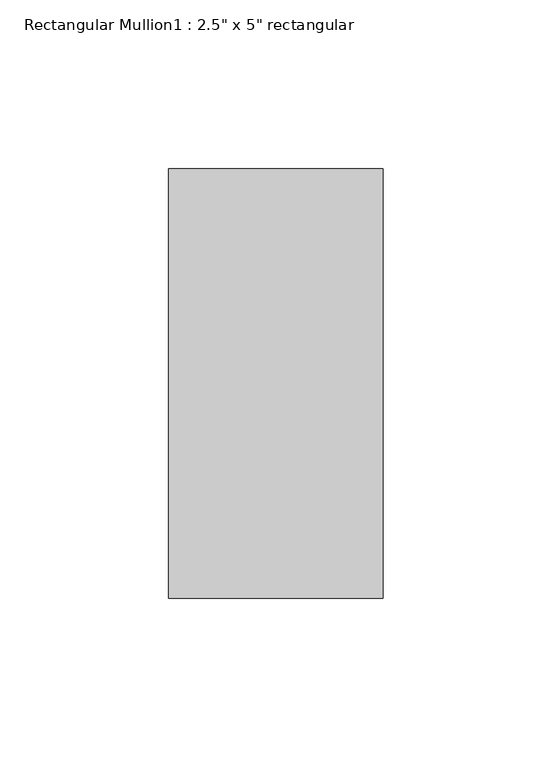
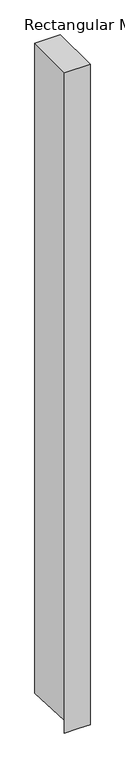
"""IFC4 building model written with IfcOpenShell, lengths in millimetres: member geometry."""

import ifcopenshell
import ifcopenshell.guid

model = None  # the IFC model being written
_history = None  # IfcOwnerHistory: only IFC2X3 demands one
_inside = {}  # id of a spatial element -> (the spatial element, [elements in it])
_under = {}  # id of a project, library or spatial element -> (it, [spatial elements below it])
_declared = {}  # id of a project -> (the project, [libraries it declares])
_typed = {}  # id of a type object -> (the type object, [elements of that type])
_made_of = {}  # id of a material, layer set ... -> (it, [elements and type objects made of it])


def new_model(schema):
    """Start an empty IFC model of exactly this schema.

    Asked for "IFC4X3", IfcOpenShell would pick the latest addendum, in which some entities
    have other attributes; the version numbers below select the first issue.
    IFC2X3 requires an IfcOwnerHistory on every rooted entity: one is made here for all.
    """
    global model, _history
    if schema == "IFC4X3":
        model = ifcopenshell.file(schema_version=(4, 3, 0, 0))
    else:
        model = ifcopenshell.file(schema=schema)
    _inside.clear()
    _under.clear()
    _declared.clear()
    _typed.clear()
    _made_of.clear()
    _history = None
    if model.schema == "IFC2X3":
        org = make("IfcOrganization", Name="unknown")
        user = make(
            "IfcPersonAndOrganization",
            ThePerson=make("IfcPerson", FamilyName="unknown"),
            TheOrganization=org,
        )
        app = make(
            "IfcApplication",
            ApplicationDeveloper=org,
            Version="unknown",
            ApplicationFullName="unknown",
            ApplicationIdentifier="unknown",
        )
        _history = make(
            "IfcOwnerHistory",
            OwningUser=user,
            OwningApplication=app,
            ChangeAction="ADDED",
            CreationDate=0,
        )
    return model


def make(cls, **values):
    """One entity of the class cls with the attributes given. An attribute that is None is left unset."""
    return model.create_entity(
        cls, **{name: value for name, value in values.items() if value is not None}
    )


def rooted(cls, **values):
    """An entity with a GlobalId (a new one), such as an element, a storey or a relation."""
    return make(cls, GlobalId=ifcopenshell.guid.new(), OwnerHistory=_history, **values)


def si_unit(unit_type, name, prefix=None):
    """IfcSIUnit, for example si_unit("LENGTHUNIT", "METRE", prefix="MILLI")."""
    return make("IfcSIUnit", UnitType=unit_type, Prefix=prefix, Name=name)


def assignment(units):
    """IfcUnitAssignment: the units of a project."""
    return None if units is None else make("IfcUnitAssignment", Units=units)


def point(xyz):
    """IfcCartesianPoint."""
    return None if xyz is None else make("IfcCartesianPoint", Coordinates=xyz)


def direction(xyz):
    """IfcDirection."""
    return None if xyz is None else make("IfcDirection", DirectionRatios=xyz)


def frame(location, z_axis=None, x_axis=None):
    """IfcAxis2Placement3D, a coordinate frame: its origin and axes. An axis left out is left unset."""
    return make(
        "IfcAxis2Placement3D",
        Location=point(location),
        Axis=direction(z_axis),
        RefDirection=direction(x_axis),
    )


def origin():
    """The frame at (0, 0, 0) with its axes left unset."""
    return frame((0.0, 0.0, 0.0))


def place(relative_to, where):
    """IfcLocalPlacement: puts the frame where relative to a parent placement (None: the world)."""
    return make(
        "IfcLocalPlacement", PlacementRelTo=relative_to, RelativePlacement=where
    )


def context(
    kind, dimensions, precision=None, world=None, true_north=None, identifier=None
):
    """IfcGeometricRepresentationContext, for example the 3D "Model" context."""
    return make(
        "IfcGeometricRepresentationContext",
        ContextIdentifier=identifier,
        ContextType=kind,
        CoordinateSpaceDimension=dimensions,
        Precision=precision,
        WorldCoordinateSystem=world,
        TrueNorth=true_north,
    )


def project(units=None, contexts=None):
    """IfcProject with its units and contexts."""
    return rooted(
        "IfcProject",
        Name="project",
        RepresentationContexts=contexts,
        UnitsInContext=assignment(units),
    )


def spatial(cls, under=None, at=None, **own):
    """A site, building, storey or space (cls), placed at a placement, below another one or the project."""
    s = rooted(cls, ObjectPlacement=at, **own)
    if under is not None:
        _under.setdefault(under.id(), (under, []))[1].append(s)
    return s


def faces_of(points, faces, orient=None, outer=None):
    """IfcFace entities. A face is a list of loops; a loop is a list of indices into points, from 0.

    orient and outer hold one flag for each loop. By default every Orientation is true, the
    first loop of a face is its IfcFaceOuterBound and the others are IfcFaceBound.
    """
    made = []
    for i, loops in enumerate(faces):
        bounds = []
        for j, loop in enumerate(loops):
            is_outer = j == 0 if outer is None else outer[i][j]
            bounds.append(
                make(
                    "IfcFaceOuterBound" if is_outer else "IfcFaceBound",
                    Bound=make("IfcPolyLoop", Polygon=[points[k] for k in loop]),
                    Orientation=True if orient is None else orient[i][j],
                )
            )
        made.append(make("IfcFace", Bounds=bounds))
    return made


def faceted_brep(points, faces, orient=None, outer=None, voids=None):
    """IfcFacetedBrep: a solid bounded by flat faces; with voids (closed shells), ...WithVoids."""
    shared = [point(p) for p in points]
    hull = make("IfcClosedShell", CfsFaces=faces_of(shared, faces, orient, outer))
    if voids is None:
        return make("IfcFacetedBrep", Outer=hull)
    return make(
        "IfcFacetedBrepWithVoids",
        Outer=hull,
        Voids=[
            make(cls, CfsFaces=faces_of(shared, fs, o, b)) for cls, fs, o, b in voids
        ],
    )


def shape(context_of_items, identifier, shape_type, items):
    """IfcShapeRepresentation: the items that make up one representation, for example the "Body"."""
    return make(
        "IfcShapeRepresentation",
        ContextOfItems=context_of_items,
        RepresentationIdentifier=identifier,
        RepresentationType=shape_type,
        Items=items,
    )


def source(mapping_origin, context_of_items, identifier, shape_type, items):
    """IfcRepresentationMap: a shape defined once, which mapped items show again and again."""
    return make(
        "IfcRepresentationMap",
        MappingOrigin=mapping_origin,
        MappedRepresentation=shape(context_of_items, identifier, shape_type, items),
    )


def transform(
    local_origin,
    x_axis=None,
    y_axis=None,
    z_axis=None,
    scale=None,
    scale2=None,
    scale3=None,
    uniform=True,
):
    """IfcCartesianTransformationOperator3D, or its non-uniform kind. x_axis, y_axis, z_axis: its Axis1, 2, 3."""
    if uniform:
        return make(
            "IfcCartesianTransformationOperator3D",
            Axis1=direction(x_axis),
            Axis2=direction(y_axis),
            LocalOrigin=point(local_origin),
            Scale=scale,
            Axis3=direction(z_axis),
        )
    return make(
        "IfcCartesianTransformationOperator3DnonUniform",
        Axis1=direction(x_axis),
        Axis2=direction(y_axis),
        LocalOrigin=point(local_origin),
        Scale=scale,
        Axis3=direction(z_axis),
        Scale2=scale2,
        Scale3=scale3,
    )


def mapped(mapping_source, mapping_target):
    """IfcMappedItem: shows the shape of a source again, moved by a transform."""
    return make(
        "IfcMappedItem", MappingSource=mapping_source, MappingTarget=mapping_target
    )


def made_of(thing, what):
    """Note that an element or type object is made of a material, layer set ...; save() writes the relation."""
    if what is not None:
        _made_of.setdefault(what.id(), (what, []))[1].append(thing)
    return thing


def element(
    cls,
    number,
    at=None,
    inside=None,
    cuts=None,
    type_object=None,
    material=None,
    context=None,
    identifier="Body",
    shape_type=None,
    held_by="IfcProductDefinitionShape",
    body=None,
    shapes=None,
    **own,
):
    """One element of the class cls, such as IfcWall. Its Tag is "e" and its number.

    at: its placement. inside: the storey or other place that contains it. cuts: it is an
    opening in that element (IfcRelVoidsElement). A single representation is given by context,
    identifier, shape_type and body (its items); several are given by shapes. held_by: the class
    of the entity that holds the representations. save() writes the other relations.
    """
    e = rooted(cls, Tag="e%d" % number, ObjectPlacement=at, **own)
    if body is not None:
        shapes = [shape(context, identifier, shape_type, body)]
    if shapes is not None:
        e.Representation = make(held_by, Representations=shapes)
    if inside is not None:
        _inside.setdefault(inside.id(), (inside, []))[1].append(e)
    if cuts is not None:
        rooted(
            "IfcRelVoidsElement", RelatingBuildingElement=cuts, RelatedOpeningElement=e
        )
    if type_object is not None:
        _typed.setdefault(type_object.id(), (type_object, []))[1].append(e)
    return made_of(e, material)


def aggregate(whole, parts):
    """IfcRelAggregates: a whole, such as a stair, and the parts it consists of."""
    return rooted("IfcRelAggregates", RelatingObject=whole, RelatedObjects=parts)


def save(model, path):
    """Write the relations noted so far, then the file.

    IfcRelAggregates (storeys below a building ...), IfcRelContainedInSpatialStructure (elements
    in a storey), IfcRelDefinesByType, IfcRelAssociatesMaterial and IfcRelDeclares: one each for
    every whole, place, type object, material and project.
    """
    for whole, parts in _under.values():
        aggregate(whole, parts)
    for where, things in _inside.values():
        rooted(
            "IfcRelContainedInSpatialStructure",
            RelatedElements=things,
            RelatingStructure=where,
        )
    for kind, things in _typed.values():
        rooted("IfcRelDefinesByType", RelatedObjects=things, RelatingType=kind)
    for what, things in _made_of.values():
        rooted("IfcRelAssociatesMaterial", RelatedObjects=things, RelatingMaterial=what)
    for by, libraries in _declared.values():
        rooted("IfcRelDeclares", RelatingContext=by, RelatedDefinitions=libraries)
    model.write(path)


def member_fbbd287a(model_context):
    return source(origin(), model_context, "Body", "Brep", [
        faceted_brep([(31.75, 63.5, 0.0), (-31.75, 63.5, 0.0), (-31.75, -63.5, 0.0), (31.75, -63.5, 0.0), (31.75, 63.5, -1705.0231573), (0.0, 63.5, -1705.0231573), (-31.75, 63.5, -1705.0231573), (-31.75, -62.1974623, -1700.0584389), (-31.75, -63.5, -1733.0362781), (0.0, -63.5, -1733.0362781), (31.75, -63.5, -1733.0362781), (31.75, -62.1974623, -1700.0584389), (0.0, -62.1974623, -1700.0584389)], [[[0, 1, 2, 3]], [[1, 0, 4, 5, 6]], [[2, 1, 6, 7, 8]], [[3, 2, 8, 9, 10]], [[0, 3, 10, 11, 4]], [[4, 11, 12, 5]], [[11, 10, 9, 12]], [[9, 8, 7, 12]], [[7, 6, 5, 12]]]),
    ])


if __name__ == "__main__":
    model = new_model("IFC4")
    model_context = context("Model", 3, world=origin())
    ifc_project = project(units=[si_unit("LENGTHUNIT", "METRE", prefix="MILLI")], contexts=[model_context])
    site = spatial("IfcSite", under=ifc_project)
    building = spatial("IfcBuilding", under=site)
    placement = place(None, origin())
    member_shape = member_fbbd287a(model_context)
    element("IfcMember", 1, ObjectType="Rectangular Mullion1 : 2.5\" x 5\" rectangular", at=placement, inside=building, context=model_context, shape_type="MappedRepresentation", body=[
        mapped(member_shape, transform((0.0, 0.0, 0.0), x_axis=(1.0, 0.0, 0.0), y_axis=(0.0, 1.0, 0.0), z_axis=(0.0, 0.0, 1.0))),
    ])
    save(model, "model.ifc")

# Revit data of these elements
# Type "Rectangular Mullion1 : 2.5\" x 5\" rectangular"
#   built-in parameter 1007304 = 0.416667 (stored number, unit not read)
#   built-in parameter 1007301 = 0.104167 (stored number, unit not read)
#   built-in parameter 1007300 = 0.104167 (stored number, unit not read)
# Element 1 (IfcMember, "Rectangular Mullion1 : 2.5\" x 5\" rectangular")
#   Materials on its faces: "support-frame"
# Materials
#   "support-frame": class "Unassigned", colour RGB 233 233 233, transparency 0, Cost = 0
